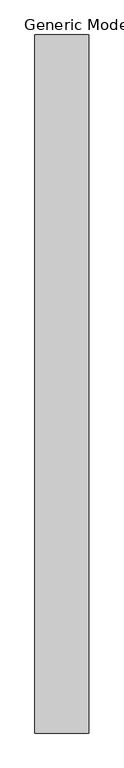
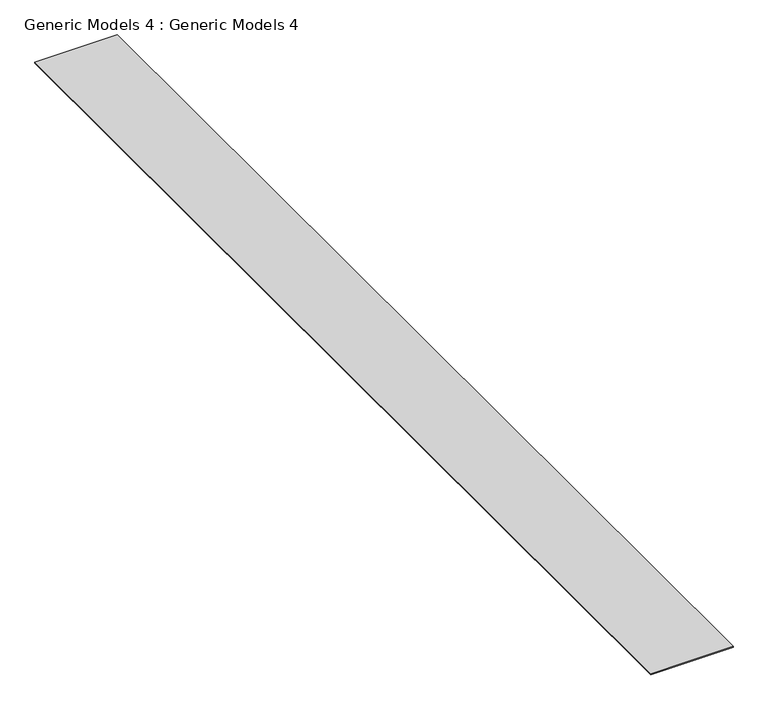
"""IFC4 building model written with IfcOpenShell, lengths in millimetres: proxy geometry, Generic Models 4 : Generic Models 4."""

from ifc_helpers import new_model, si_unit, frame, origin, place, context, project, spatial, polyline, outline, extrude, source, transform, mapped, element, save


def generic_models_4_generic_models_4_cecf207e(model_context):
    return source(origin(), model_context, "Body", "SweptSolid", [
        extrude(outline(polyline([(8575.5013705, -6864.9230338), (7140.4013705, -6864.9230338), (7140.4013705, 11778.6769662), (8575.5013705, 11778.6769662), (8575.5013705, -6864.9230338)])), frame((0.0, 0.0, 126771.146), z_axis=(0.0, 0.0, 1.0), x_axis=(1.0, 0.0, 0.0)), (0.0, 0.0, 1.0), 19.05),
    ])


if __name__ == "__main__":
    model = new_model("IFC4")
    model_context = context("Model", 3, world=origin())
    ifc_project = project(units=[si_unit("LENGTHUNIT", "METRE", prefix="MILLI")], contexts=[model_context])
    site = spatial("IfcSite", under=ifc_project)
    building = spatial("IfcBuilding", under=site)
    placement = place(None, origin())
    generic_models_4_generic_models_4_shape = generic_models_4_generic_models_4_cecf207e(model_context)
    element("IfcBuildingElementProxy", 1, Name="Generic Models 4 : Generic Models 4", ObjectType="Generic Models 4 : Generic Models 4", at=placement, inside=building, context=model_context, shape_type="MappedRepresentation", body=[
        mapped(generic_models_4_generic_models_4_shape, transform((0.0, 0.0, 0.0), x_axis=(1.0, 0.0, 0.0), y_axis=(0.0, 1.0, 0.0), z_axis=(0.0, 0.0, 1.0))),
    ])
    save(model, "model.ifc")

# Revit data of these elements
# Element 1 (IfcBuildingElementProxy, "Generic Models 4 : Generic Models 4")
#   Materials on its faces: "_CDX PLYWOOD - SEE STRUCT DWGs"
# Materials
#   "_CDX PLYWOOD - SEE STRUCT DWGs": class "Generic", colour RGB 98 75 74, transparency 0, Cost = 0
